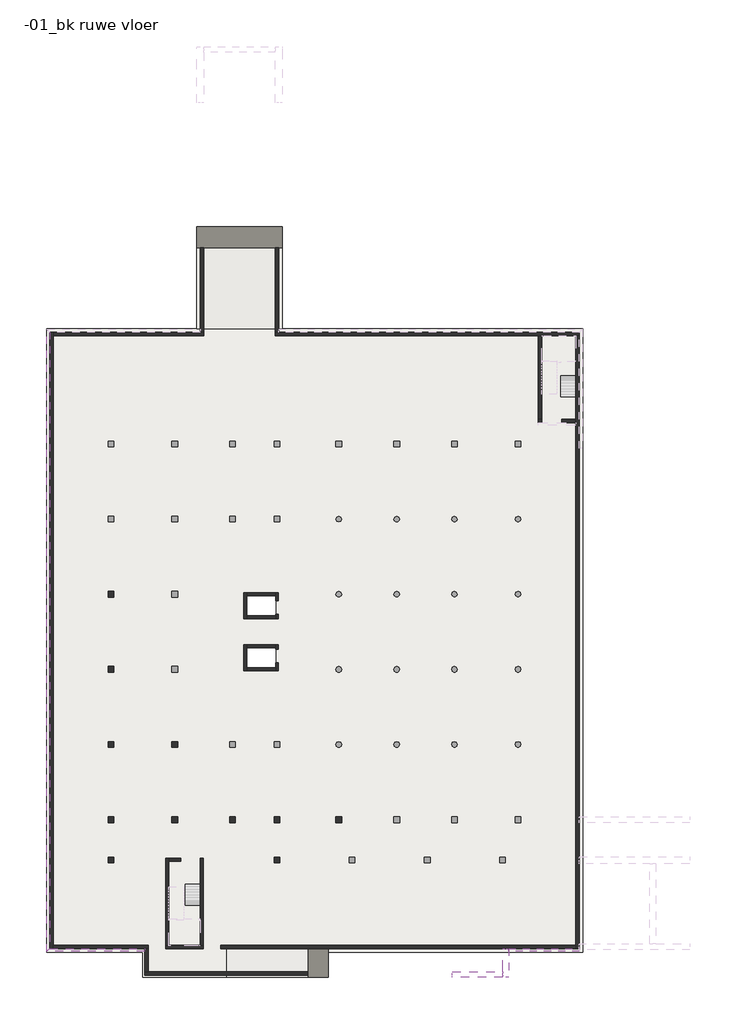
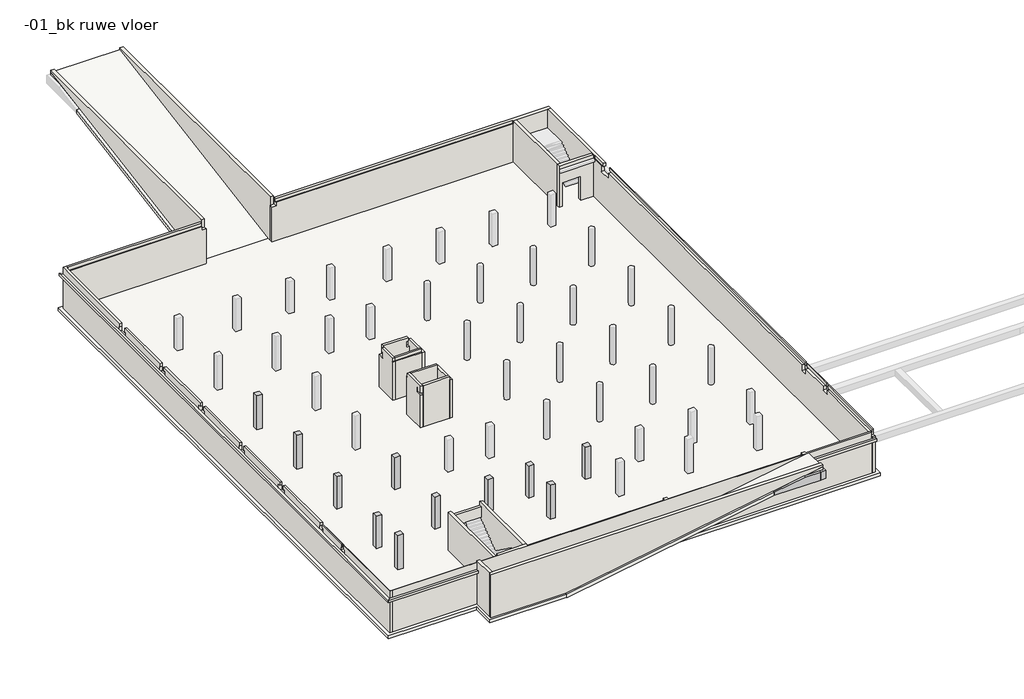
# One storey, part 1 of 2: 25 walls, 12 footings, 11 columns, 3 slabs, 2 beams.
# Revit data of these elements (continued)
# Grids (mm) (continued)
#   "I": line (-1553.97, 45500) -> (77731.283, 45500)
#   "L": line (13000, -4030.51) -> (13000, 79064.564)
# Type "NLRS_16_SF_LIB_funderingsbalk beton ihwg-CWV-MMBC-SRP_gen_rsf : funderingsbalk beton ihwg_gen__bxh 500x800"
#   Type IfcGUID = "3yoae3mAzBRekDMiYpsxNi"
#   IfcExportAs = "IfcBeamType"
#   Type Comments = "500x800"
#   Model = "LOD300"
#   Description = "funderingsbalk beton ihwg 500x800"
#   Assembly Code = "16.12"
#   NLRS_C_lengte [instance default] = 3000 mm
#   NLRS_C_hoogte = 800 mm
#   NLRS_C_breedte = 500 mm
#   Length [instance default] = 3000 mm
#   Structural Material = NLRS_f2_beton ihwg_gen_rsf
# Type "NLRS_28_SCO_TLB_vierkante kolom beton prefab-BCPG-MMBPC-SRP_gen_rsf : kolom vierkant beton prefab_gen__bxh 500x500"
#   Type IfcGUID = "2bNskL0kfByRmbY5G6If6v"
#   IfcExportAs = "IfcColumnType"
#   IfcExportType = "COLUMN"
#   Type Comments = "500x500"
#   Description = "prefab betonkolom 500x500"
#   Assembly Code = "28.11"
#   NLRS_C_lengte [instance default] = 2700 mm
#   NLRS_C_hoogte = 500 mm
#   NLRS_C_breedte = 500 mm
#   Structural Material = NLRS_f2_beton prefab_gen_rsf
#   Model = ""
# Type "NLRS_16_SFO_LB_funderingspoer meerpaals beton ihwg-MMBC-SH_gen_rsf : funderingspoer beton ihwg_gen__4-paals bxlxh 1800x1800x1200"
#   IfcExportAs = "IfcFootingType"
#   Type Comments = "4-paals poer 1800x1800x1200"
#   Model = " "
#   Manufacturer = " "
#   Keynote = "4-paals poer 1800x1800x1200"
#   Description = "4-paals poer 1800x1800x1200"
#   Assembly Code = "16.13"
#   Width = 1800 mm
#   Rough Height = 1200 mm
#   NLRS_C_lengte = 1800 mm
#   NLRS_C_hoogte = 1200 mm
#   NLRS_C_breedte = 1800 mm
#   Length = 1800 mm
#   Height [instance default] = 1050 mm
#   Foundation Thickness = 1200 mm
#   Depth [instance default] = 150 mm
#   Structural Material = NLRS_f2_beton ihwg_gen_rsf
# Type "NLRS_16_SFO_LB_funderingspoer meerpaals beton ihwg-MMBC-SH_gen_rsf : funderingspoer beton ihwg_gen__3-paals bxlxh 1800x1800x1200"
#   IfcExportAs = "IfcFootingType"
#   Type Comments = "3-paals poer 1800x1800x1200"
#   Model = " "
#   Manufacturer = " "
#   Description = "3-paals poer 1800x1800x1200"
#   Assembly Code = "16.13"
#   Width = 1800 mm
#   Rough Height = 1200 mm
#   NLRS_C_lengte = 1800 mm
#   NLRS_C_hoogte = 1200 mm
#   NLRS_C_breedte = 1800 mm
#   Length = 1800 mm
#   Height [instance default] = 1050 mm
#   Foundation Thickness = 1200 mm
#   Depth [instance default] = 150 mm
#   Structural Material = NLRS_f2_beton ihwg_gen_rsf
#   Keynote = ""
# Type "NLRS_16_SFO_LB_funderingspoer meerpaals beton ihwg-MMBC-SH_gen_rsf : funderingspoer beton ihwg_gen__2-paals bxlxh 700x1800x1200"
#   IfcExportAs = "IfcFootingType"
#   Type Comments = "2-paals poer 700x1800x1200"
#   Model = " "
#   Manufacturer = " "
#   Description = "2-paals poer 700x1800x1200"
#   Assembly Code = "16.13"
#   Width = 700 mm
#   Rough Height = 1200 mm
#   NLRS_C_lengte = 1800 mm
#   NLRS_C_hoogte = 1200 mm
#   NLRS_C_breedte = 700 mm
#   Length = 1800 mm
#   Height [instance default] = 1050 mm
#   Foundation Thickness = 1200 mm
#   Depth [instance default] = 150 mm
#   Structural Material = NLRS_f2_beton ihwg_gen_rsf
#   Keynote = ""
# Type "NLRS_16_SFO_LB_funderingspoer meerpaals beton ihwg-MMBC-SH_gen_rsf : funderingspoer beton ihwg_gen__1-paals bxlxh 700x700x500"
#   IfcExportAs = "IfcFootingType"
#   Type Comments = "1-paals poer 700x700x500"
#   Model = " "
#   Manufacturer = " "
#   Description = "1-paals poer 700x700x500"
#   Assembly Code = "16.13"
#   Width = 700 mm
#   Rough Height = 500 mm
#   NLRS_C_lengte = 700 mm
#   NLRS_C_hoogte = 500 mm
#   NLRS_C_breedte = 700 mm
#   Length = 700 mm
#   Height [instance default] = 350 mm
#   Foundation Thickness = 500 mm
#   Depth [instance default] = 150 mm
#   Structural Material = NLRS_f2_beton ihwg_gen_rsf
#   Keynote = ""
# Type "NLRS_16_SFO_LB_funderingspoer meerpaals beton ihwg-MMBC-SH_gen_rsf : funderingspoer beton ihwg_gen__trap bxlxh 3800x9300x1200"
#   IfcExportAs = "IfcFootingType"
#   Type Comments = "trappenhuispoer 3800x9300x1200"
#   Model = " "
#   Manufacturer = " "
#   Keynote = "trappenhuispoer 3800x9300x1200"
#   Description = "trappenhuispoer 3800x9300x1200"
#   Assembly Code = "16.13"
#   Width = 3800 mm
#   Rough Height = 1200 mm
#   NLRS_C_lengte = 9300 mm
#   NLRS_C_hoogte = 1200 mm
#   NLRS_C_breedte = 3800 mm
#   Length = 9300 mm
#   Height [instance default] = 1050 mm
#   Foundation Thickness = 1200 mm
#   Depth [instance default] = 150 mm
#   Structural Material = NLRS_f2_beton ihwg_gen_rsf
# Type "NLRS_13_FL_beton ihwg 300_gen_rsf"
#   Keynote = ""
#   Type IfcGUID = "2Gmsv2lRH0fOa54XIbCVVz"
#   Type Comments = "d=300mm"
#   Description = "300mm in het werk gestorte betonvloer"
#   Assembly Code = "13.22"
#   IfcExportAs = "IfcSlab"
#   Function = 1
#   Layers, outside or top first: 300 mm "NLRS_f2_beton ihwg_gen_rsf" (function 1)
# Type "NLRS_16_WA_hollewand 300_gen_rsf"
#   Keynote = ""
#   Type IfcGUID = "3S13A4zHzAqApml_3w1Yzy"
#   Description = "buitenwand holle wand, generiek"
#   Assembly Code = "16.23"
#   IfcExportAs = "IfcWall"
#   Layers, outside or top first: 60 mm "NLRS_f2_beton prefab_gen_rsf" (function 1); 0 mm "NLRS_f2_beton ihwg_gen_rsf" (function 1); 60 mm "NLRS_f2_beton prefab_gen_rsf" (function 1)
# Type "NLRS_16_WA_beton ihw 300_gen_rsf"
#   Keynote = ""
#   Type IfcGUID = "3S1HfGygHC08_ZXeiJ7DHR"
#   Description = "buitenwand beton ihw, generiek"
#   Assembly Code = "16.23"
#   IfcExportAs = "IfcWall"
#   Layers, outside or top first: 300 mm "NLRS_f2_beton ihwg_gen_rsf" (function 1)
# Type "NLRS_21_WA_beton ihw 250_gen_rsf"
#   Keynote = ""
#   Type IfcGUID = "1pBmRfcsbA7BE9s_rekBP3"
#   Description = "buitenwand beton ihw, generiek"
#   Assembly Code = "21.21"
#   IfcExportAs = "IfcWall"
#   Layers, outside or top first: 250 mm "NLRS_f2_beton ihwg_gen_rsf" (function 1)
# Type "NLRS_21_WA_beton prefab 300_gen_rsf"
#   Keynote = ""
#   Type IfcGUID = "2ajLwCSRTE_9I1Spg4sCru"
#   Description = "buitenwand beton prefab, generiek"
#   Assembly Code = "21.21"
#   IfcExportAs = "IfcWall"
#   Layers, outside or top first: 300 mm "NLRS_f2_beton prefab_gen_rsf" (function 1)
# Type "NLRS_16_SF_LIB_oplegnok beton prefab framing-CWV-MMBPC-SRP_gen_rsf : oplegnok beton prefab_gen__bxh 250x250/220"
#   Type IfcGUID = "2pBZpvCtn46PjCcATwz$Ih"
#   IfcExportAs = "IfcWallType"
#   Type Comments = "oplegnok"
#   Model = "LOD300"
#   Description = "oplegnok beton prefab 250x250/220"
#   Assembly Code = "16.23"
#   NLRS_C_hoogte_01 = 220 mm
#   NLRS_C_hoogte = 250 mm
#   NLRS_C_breedte = 250 mm
#   Lossing = 30 mm
#   Length [instance default] = 3000 mm
#   Structural Material = NLRS_f2_beton prefab_gen_rsf
# Element 1 (IfcBeam, "NLRS_16_SF_LIB_funderingsbalk beton ihwg-CWV-MMBC-SRP_gen_rsf : funderingsbalk beton ihwg_gen__bxh 500x800")
#   IfcGUID = "3yoae3mAzBRekDMiYpswhz"
#   Comments = ""
#   NLRS_C_lengte = 2650 mm
#   IsExternal = yes
#   LoadBearing = yes
#   Phase Created = NLRS_nieuw
#   Materials on its faces: "NLRS_f2_beton ihwg_gen_rsf"
# Element 2 (IfcBeam, "NLRS_16_SF_LIB_funderingsbalk beton ihwg-CWV-MMBC-SRP_gen_rsf : funderingsbalk beton ihwg_gen__bxh 500x800")
#   IfcGUID = "3yoae3mAzBRekDMiYpswfN"
#   NLRS_C_lengte = 4866.131 mm
#   IsExternal = yes
#   LoadBearing = yes
#   Phase Created = NLRS_nieuw
#   Materials on its faces: "NLRS_f2_beton ihwg_gen_rsf"
# Element 3 (IfcColumn, "NLRS_28_SCO_TLB_vierkante kolom beton prefab-BCPG-MMBPC-SRP_gen_rsf : kolom vierkant beton prefab_gen__bxh 500x500")
#   IfcGUID = "2bNskL0kfByRmbY5G6If5v"
#   IsExternal = yes
#   LoadBearing = yes
#   Phase Created = NLRS_nieuw
#   Materials on its faces: "NLRS_f2_beton prefab_gen_rsf"
# Element 4 (IfcColumn, "NLRS_28_SCO_TLB_vierkante kolom beton prefab-BCPG-MMBPC-SRP_gen_rsf : kolom vierkant beton prefab_gen__bxh 500x500")
#   IfcGUID = "2bNskL0kfByRmbY5G6If62"
#   IsExternal = yes
#   LoadBearing = yes
#   Phase Created = NLRS_nieuw
#   Materials on its faces: "NLRS_f2_beton prefab_gen_rsf"
# Element 5 (IfcColumn, "NLRS_28_SCO_TLB_vierkante kolom beton prefab-BCPG-MMBPC-SRP_gen_rsf : kolom vierkant beton prefab_gen__bxh 500x500")
#   IfcGUID = "2bNskL0kfByRmbY5G6If64"
#   IsExternal = yes
#   LoadBearing = yes
#   Phase Created = NLRS_nieuw
#   Materials on its faces: "NLRS_f2_beton prefab_gen_rsf"
# Element 6 (IfcColumn, "NLRS_28_SCO_TLB_vierkante kolom beton prefab-BCPG-MMBPC-SRP_gen_rsf : kolom vierkant beton prefab_gen__bxh 500x500")
#   IfcGUID = "2bNskL0kfByRmbY5G6If9_"
#   IsExternal = yes
#   LoadBearing = yes
#   Phase Created = NLRS_nieuw
#   Materials on its faces: "NLRS_f2_beton prefab_gen_rsf"
# Element 7 (IfcColumn, "NLRS_28_SCO_TLB_vierkante kolom beton prefab-BCPG-MMBPC-SRP_gen_rsf : kolom vierkant beton prefab_gen__bxh 500x500")
#   IfcGUID = "2fqjgN40rEBBKvfwcj0BX5"
#   IsExternal = yes
#   LoadBearing = yes
#   Phase Created = NLRS_nieuw
#   Materials on its faces: "NLRS_f2_beton prefab_gen_rsf"
# Element 8 (IfcColumn, "NLRS_28_SCO_TLB_vierkante kolom beton prefab-BCPG-MMBPC-SRP_gen_rsf : kolom vierkant beton prefab_gen__bxh 500x500")
#   IfcGUID = "2r1e$qonv1u8B8mI4Mnhtx"
#   IsExternal = yes
#   LoadBearing = yes
#   Phase Created = NLRS_nieuw
#   Materials on its faces: "NLRS_f2_beton prefab_gen_rsf"
# Element 9 (IfcColumn, "NLRS_28_SCO_TLB_vierkante kolom beton prefab-BCPG-MMBPC-SRP_gen_rsf : kolom vierkant beton prefab_gen__bxh 500x500")
#   IfcGUID = "2r1e$qonv1u8B8mI4Mnhtz"
#   IsExternal = yes
#   LoadBearing = yes
#   Phase Created = NLRS_nieuw
#   Materials on its faces: "NLRS_f2_beton prefab_gen_rsf"
# Element 10 (IfcColumn, "NLRS_28_SCO_TLB_vierkante kolom beton prefab-BCPG-MMBPC-SRP_gen_rsf : kolom vierkant beton prefab_gen__bxh 500x500")
#   IfcGUID = "2r1e$qonv1u8B8mI4Mnht$"
#   IsExternal = yes
#   LoadBearing = yes
#   Phase Created = NLRS_nieuw
#   Materials on its faces: "NLRS_f2_beton prefab_gen_rsf"
# Element 11 (IfcColumn, "NLRS_28_SCO_TLB_vierkante kolom beton prefab-BCPG-MMBPC-SRP_gen_rsf : kolom vierkant beton prefab_gen__bxh 500x500")
#   IfcGUID = "2r1e$qonv1u8B8mI4Mnhtn"
#   IsExternal = yes
#   LoadBearing = yes
#   Phase Created = NLRS_nieuw
#   Materials on its faces: "NLRS_f2_beton prefab_gen_rsf"
# Element 12 (IfcColumn, "NLRS_28_SCO_TLB_vierkante kolom beton prefab-BCPG-MMBPC-SRP_gen_rsf : kolom vierkant beton prefab_gen__bxh 500x500")
#   IfcGUID = "2r1e$qonv1u8B8mI4MnhnB"
#   IsExternal = yes
#   LoadBearing = yes
#   Phase Created = NLRS_nieuw
#   Materials on its faces: "NLRS_f2_beton prefab_gen_rsf"
# Element 13 (IfcColumn, "NLRS_28_SCO_TLB_vierkante kolom beton prefab-BCPG-MMBPC-SRP_gen_rsf : kolom vierkant beton prefab_gen__bxh 500x500")
#   IfcGUID = "3oP0NMpTfAUg2$4DiBSKtG"
#   IsExternal = yes
#   LoadBearing = yes
#   Phase Created = NLRS_nieuw
#   Materials on its faces: "NLRS_f2_beton prefab_gen_rsf"
# Element 14 (IfcFooting, "NLRS_16_SFO_LB_funderingspoer meerpaals beton ihwg-MMBC-SH_gen_rsf : funderingspoer beton ihwg_gen__4-paals bxlxh 1800x1800x1200")
#   IfcGUID = "1GXoSzV6T12eGHLrhjoRHH"
#   Height = 900 mm
#   Depth = 300 mm
#   IsExternal = yes
#   LoadBearing = yes
#   Phase Created = NLRS_nieuw
#   Materials on its faces: "NLRS_f2_beton ihwg_gen_rsf"
# Element 15 (IfcFooting, "NLRS_16_SFO_LB_funderingspoer meerpaals beton ihwg-MMBC-SH_gen_rsf : funderingspoer beton ihwg_gen__3-paals bxlxh 1800x1800x1200")
#   IfcGUID = "1GXoSzV6T12eGHLrhjoRH8"
#   Height = 900 mm
#   Depth = 300 mm
#   IsExternal = yes
#   LoadBearing = yes
#   Phase Created = NLRS_nieuw
#   Materials on its faces: "NLRS_f2_beton ihwg_gen_rsf"
# Element 16 (IfcFooting, "NLRS_16_SFO_LB_funderingspoer meerpaals beton ihwg-MMBC-SH_gen_rsf : funderingspoer beton ihwg_gen__2-paals bxlxh 700x1800x1200")
#   IfcGUID = "1GXoSzV6T12eGHLrhjoRHh"
#   Height = 900 mm
#   Depth = 300 mm
#   IsExternal = yes
#   LoadBearing = yes
#   Phase Created = NLRS_nieuw
#   Materials on its faces: "NLRS_f2_beton ihwg_gen_rsf"
# Element 17 (IfcFooting, "NLRS_16_SFO_LB_funderingspoer meerpaals beton ihwg-MMBC-SH_gen_rsf : funderingspoer beton ihwg_gen__2-paals bxlxh 700x1800x1200")
#   IfcGUID = "1GXoSzV6T12eGHLrhjoRVg"
#   Height = 900 mm
#   Depth = 300 mm
#   IsExternal = yes
#   LoadBearing = yes
#   Phase Created = NLRS_nieuw
#   Materials on its faces: "NLRS_f2_beton ihwg_gen_rsf"
# Element 18 (IfcFooting, "NLRS_16_SFO_LB_funderingspoer meerpaals beton ihwg-MMBC-SH_gen_rsf : funderingspoer beton ihwg_gen__2-paals bxlxh 700x1800x1200")
#   IfcGUID = "1GXoSzV6T12eGHLrhjoRST"
#   Height = 900 mm
#   Depth = 300 mm
#   IsExternal = yes
#   LoadBearing = yes
#   Phase Created = NLRS_nieuw
#   Materials on its faces: "NLRS_f2_beton ihwg_gen_rsf"
# Element 19 (IfcFooting, "NLRS_16_SFO_LB_funderingspoer meerpaals beton ihwg-MMBC-SH_gen_rsf : funderingspoer beton ihwg_gen__1-paals bxlxh 700x700x500")
#   IfcGUID = "1GXoSzV6T12eGHLrhjoRSM"
#   Height = 200 mm
#   Depth = 300 mm
#   IsExternal = yes
#   LoadBearing = yes
#   Phase Created = NLRS_nieuw
#   Materials on its faces: "NLRS_f2_beton ihwg_gen_rsf"
# Element 20 (IfcFooting, "NLRS_16_SFO_LB_funderingspoer meerpaals beton ihwg-MMBC-SH_gen_rsf : funderingspoer beton ihwg_gen__1-paals bxlxh 700x700x500")
#   IfcGUID = "1GXoSzV6T12eGHLrhjoRS9"
#   Height = 200 mm
#   Depth = 300 mm
#   IsExternal = yes
#   LoadBearing = yes
#   Phase Created = NLRS_nieuw
#   Materials on its faces: "NLRS_f2_beton ihwg_gen_rsf"
# Element 21 (IfcFooting, "NLRS_16_SFO_LB_funderingspoer meerpaals beton ihwg-MMBC-SH_gen_rsf : funderingspoer beton ihwg_gen__1-paals bxlxh 700x700x500")
#   IfcGUID = "1GXoSzV6T12eGHLrhjoRTF"
#   Height = 200 mm
#   Depth = 300 mm
#   IsExternal = yes
#   LoadBearing = yes
#   Phase Created = NLRS_nieuw
#   Materials on its faces: "NLRS_f2_beton ihwg_gen_rsf"
# Element 22 (IfcFooting, "NLRS_16_SFO_LB_funderingspoer meerpaals beton ihwg-MMBC-SH_gen_rsf : funderingspoer beton ihwg_gen__2-paals bxlxh 700x1800x1200")
#   IfcGUID = "3VXE8Tiz5F69n85q0kAzIM"
#   Height = 900 mm
#   Depth = 300 mm
#   IsExternal = yes
#   LoadBearing = yes
#   Phase Created = NLRS_nieuw
#   Materials on its faces: "NLRS_f2_beton ihwg_gen_rsf"
# Element 23 (IfcFooting, "NLRS_16_SFO_LB_funderingspoer meerpaals beton ihwg-MMBC-SH_gen_rsf : funderingspoer beton ihwg_gen__4-paals bxlxh 1800x1800x1200")
#   IfcGUID = "3Qemsd6Xj1WRJeMYmB12n_"
#   Height = 900 mm
#   Depth = 300 mm
#   IsExternal = yes
#   LoadBearing = yes
#   Phase Created = NLRS_nieuw
#   Materials on its faces: "NLRS_f2_beton ihwg_gen_rsf"
# Element 24 (IfcFooting, "NLRS_16_SFO_LB_funderingspoer meerpaals beton ihwg-MMBC-SH_gen_rsf : funderingspoer beton ihwg_gen__trap bxlxh 3800x9300x1200")
#   IfcGUID = "3Qemsd6Xj1WRJeMYmB12_u"
#   Height = 900 mm
#   Depth = 300 mm
#   IsExternal = yes
#   LoadBearing = yes
#   Phase Created = NLRS_nieuw
#   Materials on its faces: "NLRS_f2_beton ihwg_gen_rsf"
# Element 25 (IfcFooting, "NLRS_16_SFO_LB_funderingspoer meerpaals beton ihwg-MMBC-SH_gen_rsf : funderingspoer beton ihwg_gen__3-paals bxlxh 1800x1800x1200")
#   IfcGUID = "3loy75XKz2Rw4dS8JWiauh"
#   Height = 900 mm
#   Depth = 300 mm
#   IsExternal = yes
#   LoadBearing = yes
#   Phase Created = NLRS_nieuw
#   Materials on its faces: "NLRS_f2_beton ihwg_gen_rsf"
# Element 26 (IfcSlab, "NLRS_13_FL_beton ihwg 300_gen_rsf")
#   IfcGUID = "2Gmsv2lRH0fOa54XIbCVVL"
#   Height Offset From Level = 0 mm
#   built-in parameter 1001954 = 1
#   IsExternal = yes
#   LoadBearing = yes
#   Phase Created = NLRS_nieuw
#   Materials on its faces: "NLRS_f2_beton ihwg_gen_rsf"
# Element 27 (IfcSlab, "NLRS_13_FL_beton ihwg 300_gen_rsf")
#   IfcGUID = "2Gmsv2lRH0fOa54XIbCUXg"
#   built-in parameter 1001955 = 3.14159 (stored number, unit not read)
#   Height Offset From Level = 0 mm
#   built-in parameter 1001954 = 1
#   IsExternal = yes
#   LoadBearing = yes
#   Phase Created = NLRS_nieuw
#   Materials on its faces: "NLRS_f2_beton ihwg_gen_rsf"
# Element 28 (IfcSlab, "NLRS_13_FL_beton ihwg 300_gen_rsf")
#   IfcGUID = "26lVpBsBf2MQJTQGM8Ms4Y"
#   Comments = ""
#   Height Offset From Level = 0 mm
#   built-in parameter 1001954 = 1
#   IsExternal = yes
#   LoadBearing = yes
#   Phase Created = NLRS_nieuw
#   Materials on its faces: "NLRS_f2_beton ihwg_gen_rsf"
# Element 29 (IfcWall, "NLRS_16_WA_hollewand 300_gen_rsf")
#   IfcGUID = "3S13A4zHzAqApml_3w1Ywi"
#   Comments = ""
#   Top Offset = 0 mm
#   Base Offset = 0 mm
#   wall height = 4130 mm
#   IsExternal = yes
#   LoadBearing = yes
#   Phase Created = NLRS_nieuw
#   Base Constraint = -01_bk ruwe vloer
#   Top Constraint = 00_bk ruwe vloer
#   Materials on its faces: "NLRS_f2_beton_prefab_gen", "NLRS_f2_beton_ihwg_gen", "NLRS_f2_beton ihwg_gen_rsf"
# Element 30 (IfcWall, "NLRS_16_WA_hollewand 300_gen_rsf")
#   IfcGUID = "2QVj0Ej6XCV9jwcNWznZWx"
#   Comments = ""
#   Top Offset = 0 mm
#   Base Offset = 0 mm
#   wall height = 4130 mm
#   IsExternal = yes
#   LoadBearing = yes
#   Phase Created = NLRS_nieuw
#   Base Constraint = -01_bk ruwe vloer
#   Top Constraint = 00_bk ruwe vloer
#   Materials on its faces: "NLRS_f2_beton ihwg_gen_rsf", "NLRS_f2_beton_ihwg_gen"
# Element 31 (IfcWall, "NLRS_16_WA_hollewand 300_gen_rsf")
#   IfcGUID = "2QVj0Ej6XCV9jwcNWznZkF"
#   Comments = ""
#   Top Offset = 0 mm
#   Base Offset = 0 mm
#   wall height = 4130 mm
#   IsExternal = yes
#   LoadBearing = yes
#   Phase Created = NLRS_nieuw
#   Base Constraint = -01_bk ruwe vloer
#   Top Constraint = 00_bk ruwe vloer
#   Materials on its faces: "NLRS_f2_beton ihwg_gen_rsf", "NLRS_f2_beton_ihwg_gen"
# Element 32 (IfcWall, "NLRS_16_WA_hollewand 300_gen_rsf")
#   IfcGUID = "2QVj0Ej6XCV9jwcNWznZj0"
#   Comments = ""
#   Top Offset = 0 mm
#   Base Offset = 0 mm
#   wall height = 4130 mm
#   IsExternal = yes
#   LoadBearing = yes
#   Phase Created = NLRS_nieuw
#   Base Constraint = -01_bk ruwe vloer
#   Top Constraint = 00_bk ruwe vloer
#   Materials on its faces: "NLRS_f2_beton_prefab_gen", "NLRS_f2_beton ihwg_gen_rsf", "NLRS_f2_beton_ihwg_gen"
# Element 33 (IfcWall, "NLRS_16_WA_hollewand 300_gen_rsf")
#   IfcGUID = "2QVj0Ej6XCV9jwcNWznZhu"
#   Comments = ""
#   Top Offset = 0 mm
#   Base Offset = 0 mm
#   wall height = 4130 mm
#   IsExternal = yes
#   LoadBearing = yes
#   Phase Created = NLRS_nieuw
#   Base Constraint = -01_bk ruwe vloer
#   Top Constraint = 00_bk ruwe vloer
#   Materials on its faces: "NLRS_f2_beton ihwg_gen_rsf", "NLRS_f2_beton_ihwg_gen"
# Element 34 (IfcWall, "NLRS_16_WA_beton ihw 300_gen_rsf")
#   IfcGUID = "3S1HfGygHC08_ZXeiJ7DJS"
#   Comments = ""
#   Top Offset = 200 mm
#   Base Offset = 0 mm
#   wall height = 4330 mm
#   IsExternal = yes
#   LoadBearing = yes
#   Phase Created = NLRS_nieuw
#   Base Constraint = -01_bk ruwe vloer
#   Top Constraint = 00_bk ruwe vloer
#   Materials on its faces: "NLRS_f2_beton ihwg_gen_rsf"
# Element 35 (IfcWall, "NLRS_16_WA_beton ihw 300_gen_rsf")
#   IfcGUID = "3S1HfGygHC08_ZXeiJ7DCk"
#   Comments = ""
#   Top Offset = 200 mm
#   Base Offset = 0 mm
#   wall height = 4330 mm
#   IsExternal = yes
#   LoadBearing = yes
#   Phase Created = NLRS_nieuw
#   Base Constraint = -01_bk ruwe vloer
#   Top Constraint = 00_bk ruwe vloer
#   Materials on its faces: "NLRS_f2_beton ihwg_gen_rsf"
# Element 36 (IfcWall, "NLRS_21_WA_beton ihw 250_gen_rsf")
#   IfcGUID = "1pBmRfcsbA7BE9s_rekBNw"
#   Comments = ""
#   Top Offset = 0 mm
#   Base Offset = 0 mm
#   wall height = 3810 mm
#   IsExternal = yes
#   LoadBearing = yes
#   Phase Created = NLRS_nieuw
#   Base Constraint = -01_bk ruwe vloer
#   Top Constraint = 00_ok ruwe vloer
#   Materials on its faces: "NLRS_f2_beton ihwg_gen_rsf"
# Element 37 (IfcWall, "NLRS_21_WA_beton ihw 250_gen_rsf")
#   IfcGUID = "1pBmRfcsbA7BE9s_rekBQ8"
#   Comments = ""
#   Top Offset = 0 mm
#   Base Offset = 0 mm
#   wall height = 3810 mm
#   IsExternal = yes
#   LoadBearing = yes
#   Phase Created = NLRS_nieuw
#   Base Constraint = -01_bk ruwe vloer
#   Top Constraint = 00_ok ruwe vloer
#   Materials on its faces: "NLRS_f2_beton ihwg_gen_rsf"
# Element 38 (IfcWall, "NLRS_21_WA_beton ihw 250_gen_rsf")
#   IfcGUID = "1pBmRfcsbA7BE9s_rekBRV"
#   Top Offset = 0 mm
#   Base Offset = 0 mm
#   wall height = 4130 mm
#   IsExternal = yes
#   LoadBearing = yes
#   Phase Created = NLRS_nieuw
#   Base Constraint = -01_bk ruwe vloer
#   Top Constraint = 00_bk ruwe vloer
#   Materials on its faces: "NLRS_f2_beton ihwg_gen_rsf"
# Element 39 (IfcWall, "NLRS_21_WA_beton ihw 250_gen_rsf")
#   IfcGUID = "3iyfZByB98yevaQCZKiCIx"
#   Comments = ""
#   Top Offset = 0 mm
#   Base Offset = 0 mm
#   wall height = 4130 mm
#   IsExternal = yes
#   LoadBearing = yes
#   Phase Created = NLRS_nieuw
#   Base Constraint = -01_bk ruwe vloer
#   Top Constraint = 00_bk ruwe vloer
#   Materials on its faces: "NLRS_f2_beton ihwg_gen_rsf"
# Element 40 (IfcWall, "NLRS_21_WA_beton ihw 250_gen_rsf")
#   IfcGUID = "3iyfZByB98yevaQCZKiCGB"
#   Comments = ""
#   Top Offset = 0 mm
#   Base Offset = 0 mm
#   wall height = 4130 mm
#   IsExternal = yes
#   LoadBearing = yes
#   Phase Created = NLRS_nieuw
#   Base Constraint = -01_bk ruwe vloer
#   Top Constraint = 00_bk ruwe vloer
#   Materials on its faces: "NLRS_f2_beton ihwg_gen_rsf"
# Element 41 (IfcWall, "NLRS_21_WA_beton ihw 250_gen_rsf")
#   IfcGUID = "3iyfZByB98yevaQCZKiCGb"
#   Comments = ""
#   Top Offset = 0 mm
#   Base Offset = 0 mm
#   wall height = 4130 mm
#   IsExternal = yes
#   LoadBearing = yes
#   Phase Created = NLRS_nieuw
#   Base Constraint = -01_bk ruwe vloer
#   Top Constraint = 00_bk ruwe vloer
#   Materials on its faces: "NLRS_f2_beton ihwg_gen_rsf"
# Element 42 (IfcWall, "NLRS_21_WA_beton ihw 250_gen_rsf")
#   IfcGUID = "3iyfZByB98yevaQCZKiClS"
#   Comments = ""
#   Top Offset = 0 mm
#   Base Offset = 0 mm
#   wall height = 3810 mm
#   IsExternal = yes
#   LoadBearing = yes
#   Phase Created = NLRS_nieuw
#   Base Constraint = -01_bk ruwe vloer
#   Top Constraint = 00_ok ruwe vloer
#   Materials on its faces: "NLRS_f2_beton ihwg_gen_rsf"
# Element 43 (IfcWall, "NLRS_21_WA_beton ihw 250_gen_rsf")
#   IfcGUID = "3iyfZByB98yevaQCZKiCjh"
#   Comments = ""
#   Top Offset = 0 mm
#   Base Offset = 0 mm
#   wall height = 4130 mm
#   IsExternal = yes
#   LoadBearing = yes
#   Phase Created = NLRS_nieuw
#   Base Constraint = -01_bk ruwe vloer
#   Top Constraint = 00_bk ruwe vloer
#   Materials on its faces: "NLRS_f2_beton ihwg_gen_rsf"
# Element 44 (IfcWall, "NLRS_21_WA_beton ihw 250_gen_rsf")
#   IfcGUID = "3iyfZByB98yevaQCZKiCi9"
#   Comments = ""
#   Top Offset = 0 mm
#   Base Offset = 0 mm
#   wall height = 4130 mm
#   IsExternal = yes
#   LoadBearing = yes
#   Phase Created = NLRS_nieuw
#   Base Constraint = -01_bk ruwe vloer
#   Top Constraint = 00_bk ruwe vloer
#   Materials on its faces: "NLRS_f2_beton ihwg_gen_rsf"
# Element 45 (IfcWall, "NLRS_21_WA_beton ihw 250_gen_rsf")
#   IfcGUID = "3iyfZByB98yevaQCZKiCik"
#   Comments = ""
#   Top Offset = 0 mm
#   Base Offset = 0 mm
#   wall height = 4130 mm
#   IsExternal = yes
#   LoadBearing = yes
#   Phase Created = NLRS_nieuw
#   Base Constraint = -01_bk ruwe vloer
#   Top Constraint = 00_bk ruwe vloer
#   Materials on its faces: "NLRS_f2_beton ihwg_gen_rsf"
# Element 46 (IfcWall, "NLRS_21_WA_beton prefab 300_gen_rsf")
#   IfcGUID = "2ajLwCSRTE_9I1Spg4sCjz"
#   Comments = ""
#   built-in parameter 1001111 = 30 mm
#   Top Offset = 0 mm
#   Base Offset = 30 mm
#   wall height = 4100 mm
#   IsExternal = yes
#   LoadBearing = yes
#   Phase Created = NLRS_nieuw
#   Base Constraint = -01_bk ruwe vloer
#   Top Constraint = 00_bk ruwe vloer
#   Materials on its faces: "NLRS_f2_beton prefab_gen_rsf"
# Element 47 (IfcWall, "NLRS_21_WA_beton prefab 300_gen_rsf")
#   IfcGUID = "2ajLwCSRTE_9I1Spg4sCjn"
#   Comments = ""
#   built-in parameter 1001111 = 30 mm
#   Top Offset = 0 mm
#   Base Offset = 30 mm
#   wall height = 4100 mm
#   IsExternal = yes
#   LoadBearing = yes
#   Phase Created = NLRS_nieuw
#   Base Constraint = -01_bk ruwe vloer
#   Top Constraint = 00_bk ruwe vloer
#   Materials on its faces: "NLRS_f2_beton prefab_gen_rsf"
# Element 48 (IfcWall, "NLRS_16_SF_LIB_oplegnok beton prefab framing-CWV-MMBPC-SRP_gen_rsf : oplegnok beton prefab_gen__bxh 250x250/220")
#   IfcGUID = "2xH6lYwJzDD8CTyoTIBXLI"
#   IsExternal = yes
#   LoadBearing = yes
#   Phase Created = NLRS_nieuw
#   Materials on its faces: "NLRS_f2_beton prefab_gen_rsf"
# Element 49 (IfcWall, "NLRS_16_SF_LIB_oplegnok beton prefab framing-CWV-MMBPC-SRP_gen_rsf : oplegnok beton prefab_gen__bxh 250x250/220")
#   IfcGUID = "2xH6lYwJzDD8CTyoTIBXLo"
#   IsExternal = yes
#   LoadBearing = yes
#   Phase Created = NLRS_nieuw
#   Materials on its faces: "NLRS_f2_beton prefab_gen_rsf"
# Element 50 (IfcWall, "NLRS_21_WA_beton ihw 250_gen_rsf")
#   IfcGUID = "1YBZRJosH5dOaCCgeRHuc1"
#   Comments = ""
#   Top Offset = 0 mm
#   Base Offset = 0 mm
#   wall height = 3810 mm
#   IsExternal = yes
#   LoadBearing = yes
#   Phase Created = NLRS_nieuw
#   Base Constraint = -01_bk ruwe vloer
#   Top Constraint = 00_ok ruwe vloer
#   Materials on its faces: "NLRS_f2_beton ihwg_gen_rsf"
# Element 51 (IfcWall, "NLRS_16_WA_beton ihw 300_gen_rsf")
#   IfcGUID = "26lVpBsBf2MQJTQGM8MsEk"
#   Comments = ""
#   Top Offset = 200 mm
#   Base Offset = 0 mm
#   wall height = 4330 mm
#   IsExternal = yes
#   LoadBearing = yes
#   Phase Created = NLRS_nieuw
#   Base Constraint = -01_bk ruwe vloer
#   Top Constraint = 00_bk ruwe vloer
#   Materials on its faces: "NLRS_f2_beton ihwg_gen_rsf"
# Element 52 (IfcWall, "NLRS_16_WA_beton ihw 300_gen_rsf")
#   IfcGUID = "26lVpBsBf2MQJTQGM8MsE9"
#   Comments = ""
#   Top Offset = 200 mm
#   Base Offset = 0 mm
#   wall height = 4330 mm
#   IsExternal = yes
#   LoadBearing = yes
#   Phase Created = NLRS_nieuw
#   Base Constraint = -01_bk ruwe vloer
#   Top Constraint = 00_bk ruwe vloer
#   Materials on its faces: "NLRS_f2_beton ihwg_gen_rsf"
# Element 53 (IfcWall, "NLRS_16_SF_LIB_oplegnok beton prefab framing-CWV-MMBPC-SRP_gen_rsf : oplegnok beton prefab_gen__bxh 250x250/220")
#   IfcGUID = "3aMdMHoe12P9KDGPyaIhSi"
#   IsExternal = yes
#   LoadBearing = yes
#   Phase Created = NLRS_nieuw
#   Materials on its faces: "NLRS_f2_beton prefab_gen_rsf"
# Materials
#   "NLRS_f2_beton ihwg_gen_rsf": class "F - Niet gebakken kunststeen", colour RGB 129 133 118, transparency 0, Keynote = "f2", Manufacturer = "Revit Standards Foundation", URL = "www.revitstandards.org", Description = "beton ihwg", Cost = 0
#   "NLRS_f2_beton prefab_gen_rsf": class "F - Niet gebakken kunststeen", colour RGB 129 133 118, transparency 0, Keynote = "f2", Manufacturer = "Revit Standards Foundation", URL = "www.revitstandards.org", Description = "beton prefab", Cost = 0
#   "NLRS_f2_beton_prefab_gen": class "Concrete", colour RGB 114 115 106, transparency 0, Manufacturer = "RevitGG", URL = "www.revitgg.nl", Description = "Beton, geprefabriceerd, generiek materiaal", Cost = 0
#   "NLRS_f2_beton_ihwg_gen": class "Concrete", colour RGB 192 192 192, transparency 0, Manufacturer = "RevitGG", URL = "www.revitgg.nl", Description = "Beton, generiek materiaal", Cost = 0
